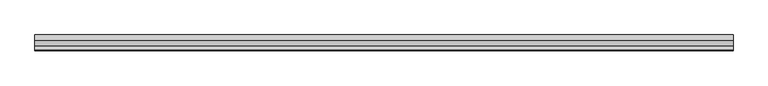
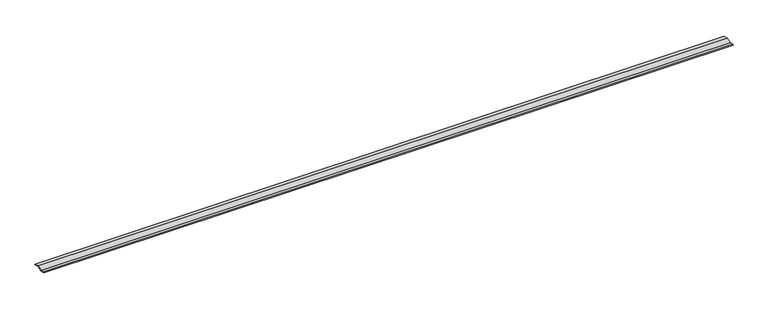
"""IFC4 building model written with IfcOpenShell, lengths in millimetres: proxy geometry, Gutter @ Roof002 : Gutter @ Roof002."""

from ifc_helpers import new_model, si_unit, frame, origin, place, context, project, spatial, polyline, outline, extrude, source, transform, mapped, element, save


def generic_models_f9d9f39b(model_context):
    return source(origin(), model_context, "Body", "SweptSolid", [
        extrude(outline(polyline([(4330.1626094, 41518.0902432), (4344.3289509, 41523.0609007), (4361.126381, 41518.7193985), (4360.4907738, 41516.260211), (4344.4411235, 41520.4084403), (4330.2808127, 41515.4398989), (4316.1841327, 41519.0141169), (4316.8083969, 41521.4762083), (4330.1626094, 41518.0902432)])), frame((255.0171875, 0.0, 0.0), z_axis=(1.0, 0.0, 0.0), x_axis=(0.0, 1.0, 0.0)), (0.0, 0.0, 1.0), 1999.85),
    ])


if __name__ == "__main__":
    model = new_model("IFC4")
    model_context = context("Model", 3, world=origin())
    ifc_project = project(units=[si_unit("LENGTHUNIT", "METRE", prefix="MILLI")], contexts=[model_context])
    site = spatial("IfcSite", under=ifc_project)
    building = spatial("IfcBuilding", under=site)
    placement = place(None, origin())
    generic_models_shape = generic_models_f9d9f39b(model_context)
    element("IfcBuildingElementProxy", 1, Name="Gutter @ Roof002 : Gutter @ Roof002", ObjectType="Gutter @ Roof002 : Gutter @ Roof002", at=placement, inside=building, context=model_context, shape_type="MappedRepresentation", body=[
        mapped(generic_models_shape, transform((0.0, 0.0, 0.0), x_axis=(1.0, 0.0, 0.0), y_axis=(0.0, 1.0, 0.0), z_axis=(0.0, 0.0, 1.0))),
    ])
    save(model, "model.ifc")

# Revit data of these elements
# Type "Gutter @ Roof002 : Gutter @ Roof002"
#   NameOverride = "Gutter @ Roof002"
# Element 1 (IfcBuildingElementProxy, "Gutter @ Roof002 : Gutter @ Roof002")
#   Materials on its faces: "CONT. SEAMLESS 16 GA COPPER BRAKE METAL GUTTER"
# Materials
#   "CONT. SEAMLESS 16 GA COPPER BRAKE METAL GUTTER": class "Unassigned", colour RGB 128 128 128, transparency 0
